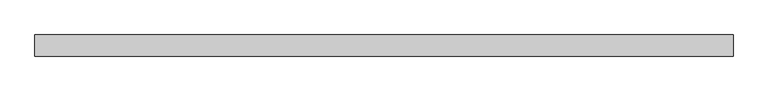
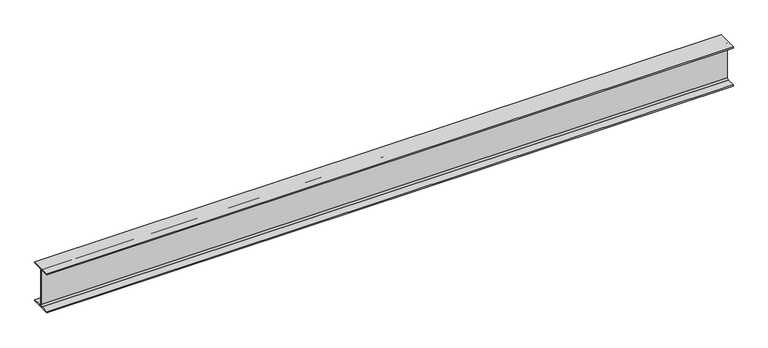
"""IFC4 building model written with IfcOpenShell, lengths in millimetres: beam geometry, 0912_Steel Framing_H-KSD3502 : H_SB_ASB_H-350x175x7x11."""

import ifcopenshell
import ifcopenshell.guid

model = None  # the IFC model being written
_history = None  # IfcOwnerHistory: only IFC2X3 demands one
_inside = {}  # id of a spatial element -> (the spatial element, [elements in it])
_under = {}  # id of a project, library or spatial element -> (it, [spatial elements below it])
_declared = {}  # id of a project -> (the project, [libraries it declares])
_typed = {}  # id of a type object -> (the type object, [elements of that type])
_made_of = {}  # id of a material, layer set ... -> (it, [elements and type objects made of it])


def new_model(schema):
    """Start an empty IFC model of exactly this schema.

    Asked for "IFC4X3", IfcOpenShell would pick the latest addendum, in which some entities
    have other attributes; the version numbers below select the first issue.
    IFC2X3 requires an IfcOwnerHistory on every rooted entity: one is made here for all.
    """
    global model, _history
    if schema == "IFC4X3":
        model = ifcopenshell.file(schema_version=(4, 3, 0, 0))
    else:
        model = ifcopenshell.file(schema=schema)
    _inside.clear()
    _under.clear()
    _declared.clear()
    _typed.clear()
    _made_of.clear()
    _history = None
    if model.schema == "IFC2X3":
        org = make("IfcOrganization", Name="unknown")
        user = make(
            "IfcPersonAndOrganization",
            ThePerson=make("IfcPerson", FamilyName="unknown"),
            TheOrganization=org,
        )
        app = make(
            "IfcApplication",
            ApplicationDeveloper=org,
            Version="unknown",
            ApplicationFullName="unknown",
            ApplicationIdentifier="unknown",
        )
        _history = make(
            "IfcOwnerHistory",
            OwningUser=user,
            OwningApplication=app,
            ChangeAction="ADDED",
            CreationDate=0,
        )
    return model


def make(cls, **values):
    """One entity of the class cls with the attributes given. An attribute that is None is left unset."""
    return model.create_entity(
        cls, **{name: value for name, value in values.items() if value is not None}
    )


def rooted(cls, **values):
    """An entity with a GlobalId (a new one), such as an element, a storey or a relation."""
    return make(cls, GlobalId=ifcopenshell.guid.new(), OwnerHistory=_history, **values)


def si_unit(unit_type, name, prefix=None):
    """IfcSIUnit, for example si_unit("LENGTHUNIT", "METRE", prefix="MILLI")."""
    return make("IfcSIUnit", UnitType=unit_type, Prefix=prefix, Name=name)


def assignment(units):
    """IfcUnitAssignment: the units of a project."""
    return None if units is None else make("IfcUnitAssignment", Units=units)


def point(xyz):
    """IfcCartesianPoint."""
    return None if xyz is None else make("IfcCartesianPoint", Coordinates=xyz)


def direction(xyz):
    """IfcDirection."""
    return None if xyz is None else make("IfcDirection", DirectionRatios=xyz)


def frame(location, z_axis=None, x_axis=None):
    """IfcAxis2Placement3D, a coordinate frame: its origin and axes. An axis left out is left unset."""
    return make(
        "IfcAxis2Placement3D",
        Location=point(location),
        Axis=direction(z_axis),
        RefDirection=direction(x_axis),
    )


def frame_2d(location, x_axis=None):
    """IfcAxis2Placement2D, a coordinate frame in the plane: its origin and x axis."""
    return make(
        "IfcAxis2Placement2D", Location=point(location), RefDirection=direction(x_axis)
    )


def origin():
    """The frame at (0, 0, 0) with its axes left unset."""
    return frame((0.0, 0.0, 0.0))


def place(relative_to, where):
    """IfcLocalPlacement: puts the frame where relative to a parent placement (None: the world)."""
    return make(
        "IfcLocalPlacement", PlacementRelTo=relative_to, RelativePlacement=where
    )


def context(
    kind, dimensions, precision=None, world=None, true_north=None, identifier=None
):
    """IfcGeometricRepresentationContext, for example the 3D "Model" context."""
    return make(
        "IfcGeometricRepresentationContext",
        ContextIdentifier=identifier,
        ContextType=kind,
        CoordinateSpaceDimension=dimensions,
        Precision=precision,
        WorldCoordinateSystem=world,
        TrueNorth=true_north,
    )


def project(units=None, contexts=None):
    """IfcProject with its units and contexts."""
    return rooted(
        "IfcProject",
        Name="project",
        RepresentationContexts=contexts,
        UnitsInContext=assignment(units),
    )


def spatial(cls, under=None, at=None, **own):
    """A site, building, storey or space (cls), placed at a placement, below another one or the project."""
    s = rooted(cls, ObjectPlacement=at, **own)
    if under is not None:
        _under.setdefault(under.id(), (under, []))[1].append(s)
    return s


def polyline(points):
    """IfcPolyline through the points."""
    return make("IfcPolyline", Points=[point(p) for p in points])


def circle_curve(where, radius):
    """IfcCircle in the frame where."""
    return make("IfcCircle", Position=where, Radius=radius)


def trimmed(basis, trim1, trim2, sense, master):
    """IfcTrimmedCurve: the piece of a basis curve between two trims."""
    return make(
        "IfcTrimmedCurve",
        BasisCurve=basis,
        Trim1=trim1,
        Trim2=trim2,
        SenseAgreement=sense,
        MasterRepresentation=master,
    )


def segment(curve, same_sense, transition):
    """IfcCompositeCurveSegment."""
    return make(
        "IfcCompositeCurveSegment",
        Transition=transition,
        SameSense=same_sense,
        ParentCurve=curve,
    )


def composite_curve(segments, self_intersect=None):
    """IfcCompositeCurve: segments joined end to end."""
    return make("IfcCompositeCurve", Segments=segments, SelfIntersect=self_intersect)


def outline(outer, holes=None, kind="AREA"):
    """IfcArbitraryClosedProfileDef: a profile drawn as a closed curve; with holes, ...WithVoids."""
    if holes is None:
        return make("IfcArbitraryClosedProfileDef", ProfileType=kind, OuterCurve=outer)
    return make(
        "IfcArbitraryProfileDefWithVoids",
        ProfileType=kind,
        OuterCurve=outer,
        InnerCurves=holes,
    )


def extrude(swept, where, along, depth):
    """IfcExtrudedAreaSolid: the profile swept, set in the frame where, extruded along a direction by depth."""
    return make(
        "IfcExtrudedAreaSolid",
        SweptArea=swept,
        Position=where,
        ExtrudedDirection=direction(along),
        Depth=depth,
    )


def shape(context_of_items, identifier, shape_type, items):
    """IfcShapeRepresentation: the items that make up one representation, for example the "Body"."""
    return make(
        "IfcShapeRepresentation",
        ContextOfItems=context_of_items,
        RepresentationIdentifier=identifier,
        RepresentationType=shape_type,
        Items=items,
    )


def source(mapping_origin, context_of_items, identifier, shape_type, items):
    """IfcRepresentationMap: a shape defined once, which mapped items show again and again."""
    return make(
        "IfcRepresentationMap",
        MappingOrigin=mapping_origin,
        MappedRepresentation=shape(context_of_items, identifier, shape_type, items),
    )


def transform(
    local_origin,
    x_axis=None,
    y_axis=None,
    z_axis=None,
    scale=None,
    scale2=None,
    scale3=None,
    uniform=True,
):
    """IfcCartesianTransformationOperator3D, or its non-uniform kind. x_axis, y_axis, z_axis: its Axis1, 2, 3."""
    if uniform:
        return make(
            "IfcCartesianTransformationOperator3D",
            Axis1=direction(x_axis),
            Axis2=direction(y_axis),
            LocalOrigin=point(local_origin),
            Scale=scale,
            Axis3=direction(z_axis),
        )
    return make(
        "IfcCartesianTransformationOperator3DnonUniform",
        Axis1=direction(x_axis),
        Axis2=direction(y_axis),
        LocalOrigin=point(local_origin),
        Scale=scale,
        Axis3=direction(z_axis),
        Scale2=scale2,
        Scale3=scale3,
    )


def mapped(mapping_source, mapping_target):
    """IfcMappedItem: shows the shape of a source again, moved by a transform."""
    return make(
        "IfcMappedItem", MappingSource=mapping_source, MappingTarget=mapping_target
    )


def made_of(thing, what):
    """Note that an element or type object is made of a material, layer set ...; save() writes the relation."""
    if what is not None:
        _made_of.setdefault(what.id(), (what, []))[1].append(thing)
    return thing


def element(
    cls,
    number,
    at=None,
    inside=None,
    cuts=None,
    type_object=None,
    material=None,
    context=None,
    identifier="Body",
    shape_type=None,
    held_by="IfcProductDefinitionShape",
    body=None,
    shapes=None,
    **own,
):
    """One element of the class cls, such as IfcWall. Its Tag is "e" and its number.

    at: its placement. inside: the storey or other place that contains it. cuts: it is an
    opening in that element (IfcRelVoidsElement). A single representation is given by context,
    identifier, shape_type and body (its items); several are given by shapes. held_by: the class
    of the entity that holds the representations. save() writes the other relations.
    """
    e = rooted(cls, Tag="e%d" % number, ObjectPlacement=at, **own)
    if body is not None:
        shapes = [shape(context, identifier, shape_type, body)]
    if shapes is not None:
        e.Representation = make(held_by, Representations=shapes)
    if inside is not None:
        _inside.setdefault(inside.id(), (inside, []))[1].append(e)
    if cuts is not None:
        rooted(
            "IfcRelVoidsElement", RelatingBuildingElement=cuts, RelatedOpeningElement=e
        )
    if type_object is not None:
        _typed.setdefault(type_object.id(), (type_object, []))[1].append(e)
    return made_of(e, material)


def aggregate(whole, parts):
    """IfcRelAggregates: a whole, such as a stair, and the parts it consists of."""
    return rooted("IfcRelAggregates", RelatingObject=whole, RelatedObjects=parts)


def save(model, path):
    """Write the relations noted so far, then the file.

    IfcRelAggregates (storeys below a building ...), IfcRelContainedInSpatialStructure (elements
    in a storey), IfcRelDefinesByType, IfcRelAssociatesMaterial and IfcRelDeclares: one each for
    every whole, place, type object, material and project.
    """
    for whole, parts in _under.values():
        aggregate(whole, parts)
    for where, things in _inside.values():
        rooted(
            "IfcRelContainedInSpatialStructure",
            RelatedElements=things,
            RelatingStructure=where,
        )
    for kind, things in _typed.values():
        rooted("IfcRelDefinesByType", RelatedObjects=things, RelatingType=kind)
    for what, things in _made_of.values():
        rooted("IfcRelAssociatesMaterial", RelatedObjects=things, RelatingMaterial=what)
    for by, libraries in _declared.values():
        rooted("IfcRelDeclares", RelatingContext=by, RelatedDefinitions=libraries)
    model.write(path)


def beam_53bde3f6(model_context):
    return source(origin(), model_context, "Body", "SweptSolid", [
        extrude(outline(composite_curve([segment(polyline([(87.5, -164.0), (87.5, -175.0), (-87.5, -175.0), (-87.5, -164.0), (-17.5, -164.0)]), True, "CONTINUOUS"), segment(trimmed(circle_curve(frame_2d((-17.5, -150.0)), 14.0), [point((-17.5, -164.0))], [point((-3.5, -150.0))], True, "CARTESIAN"), True, "CONTINUOUS"), segment(polyline([(-3.5, -150.0), (-3.5, 150.0)]), True, "CONTINUOUS"), segment(trimmed(circle_curve(frame_2d((-17.5, 150.0)), 14.0), [point((-3.5, 150.0))], [point((-17.5, 164.0))], True, "CARTESIAN"), True, "CONTINUOUS"), segment(polyline([(-17.5, 164.0), (-87.5, 164.0), (-87.5, 175.0), (87.5, 175.0), (87.5, 164.0), (17.5, 164.0)]), True, "CONTINUOUS"), segment(trimmed(circle_curve(frame_2d((17.5, 150.0)), 14.0), [point((17.5, 164.0))], [point((3.5, 150.0))], True, "CARTESIAN"), True, "CONTINUOUS"), segment(polyline([(3.5, 150.0), (3.5, -150.0)]), True, "CONTINUOUS"), segment(trimmed(circle_curve(frame_2d((17.5, -150.0)), 14.0), [point((3.5, -150.0))], [point((17.5, -164.0))], True, "CARTESIAN"), True, "CONTINUOUS"), segment(polyline([(17.5, -164.0), (87.5, -164.0)]), True, "CONTINUOUS")], self_intersect=False)), frame((-2769.2350039, 0.0, 0.0), z_axis=(1.0, 0.0, 0.0), x_axis=(0.0, 1.0, 0.0)), (0.0, 0.0, 1.0), 5784.1976903),
    ])


if __name__ == "__main__":
    model = new_model("IFC4")
    model_context = context("Model", 3, world=origin())
    ifc_project = project(units=[si_unit("LENGTHUNIT", "METRE", prefix="MILLI")], contexts=[model_context])
    site = spatial("IfcSite", under=ifc_project)
    building = spatial("IfcBuilding", under=site)
    placement = place(None, origin())
    beam_shape = beam_53bde3f6(model_context)
    element("IfcBeam", 1, ObjectType="0912_Steel Framing_H-KSD3502 : H_SB_ASB_H-350x175x7x11", at=placement, inside=building, context=model_context, shape_type="MappedRepresentation", body=[
        mapped(beam_shape, transform((0.0, 0.0, 0.0), x_axis=(1.0, 0.0, 0.0), y_axis=(0.0, 1.0, 0.0), z_axis=(0.0, 0.0, 1.0))),
    ])
    save(model, "model.ifc")

# Revit data of these elements
# Type "0912_Steel Framing_H-KSD3502 : H_SB_ASB_H-350x175x7x11"
#   H_WM Code_1 = "S01AA002-00001 | Main Steel Structure Fabrication Work | Shelter/Building | Medium Steel - Standard (90KG/M>Weight≥30KG/M) | Material: (   )"
#   H_WM Code_2 = "S03AA028-00001 | Main Steel Structure Erection Work | Shelter/Building | Medium Steel (90KG/M>Weight≥30KG/M) | Material: (   )"
#   H_WM Code_3 = "S01AA010-00001 | Main Steel Structure Fabrication Work | Shelter/Building | Steel Painting/Coating | for Non-Fireproofed Steel Surface, Surface Preparation, Primer, Second & Final Coat | Material: (   )"
#   H_Q'ty Cal Type Tag = "SB-Q2"
#   Width = 17.5 cm
#   Web Thickness = 0.7 cm
#   Web Fillet = 1.4 cm
#   Warping Constant = 282000.0 cm⁶
#   W = 0
#   Torsional Moment of Inertia = 19.4042 cm⁴
#   Section Area = 63.14 cm²
#   Plastic Modulus weak axis = 174.0 cm³
#   Plastic Modulus strong axis = 868.0 cm³
#   Perimeter = 1.36 m²/m
#   Nominal Weight = 49.60 kgf/m
#   Moment of Inertia weak axis = 984.00 cm⁴
#   Moment of Inertia strong axis = 13600.00 cm⁴
#   Height = 35.0 cm
#   Flange Thickness = 1.1 cm
#   Elastic Modulus weak axis = 112.0 cm³
#   Elastic Modulus strong axis = 775.0 cm³
#   Centroid Vertical = 17.5 cm
#   Centroid Horizontal = 8.75 cm
#   Ix = 136000000
#   Length [instance default] = 1.5240 m
#   Zx = 868000
#   b = 0.1750 m
#   h = 0.3500 m
#   r = 0.0140 m
#   s = 0.0070 m
#   t = 0.0110 m
#   A = 0.006314 m²
#   Structural Material [instance default] = Steel, 45-345
#   Assembly Code = ""
# Element 1 (IfcBeam, "0912_Steel Framing_H-KSD3502 : H_SB_ASB_H-350x175x7x11")
#   Structural Material = none
# Materials
#   "Steel, 45-345": class "Metal", colour RGB 189 187 185, transparency 0, Description = "Steel 345 MPa", Cost = 0
